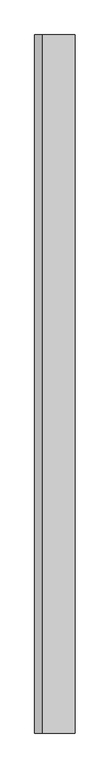
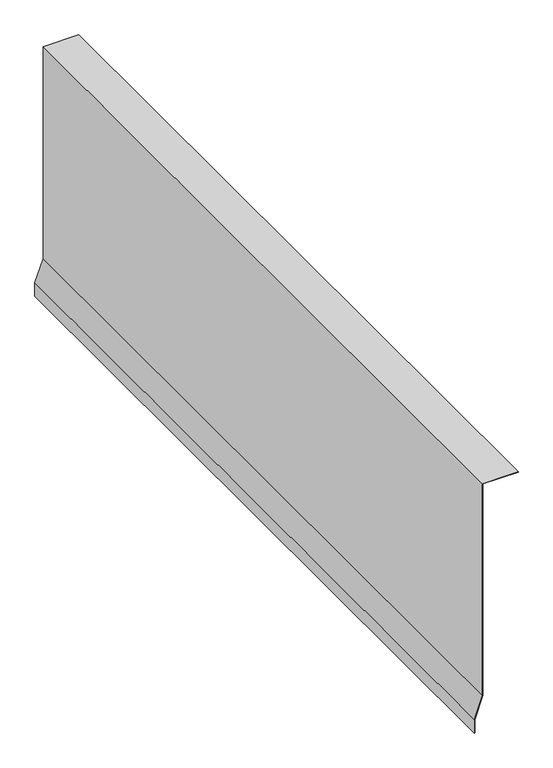
"""IFC4 building model written with IfcOpenShell, lengths in millimetres: proxy geometry, Membrane056 15639 : Membrane056 15639."""

from ifc_helpers import new_model, si_unit, frame, origin, place, context, project, spatial, polyline, outline, extrude, source, transform, mapped, element, save


def generic_models_2c707389(model_context):
    return source(origin(), model_context, "Body", "SweptSolid", [
        extrude(outline(polyline([(40237.828125, -4904.6197981), (40237.828125, -4998.1919031), (39649.4031064, -4998.1919031), (39589.4778975, -5020.0028954), (39552.6918208, -5020.0028954), (39552.6918208, -5019.0028954), (39589.3015705, -5019.0028954), (39649.2267794, -4997.1919031), (40236.828125, -4997.1919031), (40236.828125, -4904.6197981), (40237.828125, -4904.6197981)])), frame((0.0, -1052.8906574, 0.0), z_axis=(0.0, 1.0, 0.0), x_axis=(0.0, 0.0, 1.0)), (0.0, 0.0, 1.0), 2000.0),
    ])


if __name__ == "__main__":
    model = new_model("IFC4")
    model_context = context("Model", 3, world=origin())
    ifc_project = project(units=[si_unit("LENGTHUNIT", "METRE", prefix="MILLI")], contexts=[model_context])
    site = spatial("IfcSite", under=ifc_project)
    building = spatial("IfcBuilding", under=site)
    placement = place(None, origin())
    generic_models_shape = generic_models_2c707389(model_context)
    element("IfcBuildingElementProxy", 1, Name="Membrane056 15639 : Membrane056 15639", ObjectType="Membrane056 15639 : Membrane056 15639", at=placement, inside=building, context=model_context, shape_type="MappedRepresentation", body=[
        mapped(generic_models_shape, transform((0.0, 0.0, 0.0), x_axis=(1.0, 0.0, 0.0), y_axis=(0.0, 1.0, 0.0), z_axis=(0.0, 0.0, 1.0))),
    ])
    save(model, "model.ifc")

# Revit data of these elements
# Type "Membrane056 15639 : Membrane056 15639"
#   NameOverride = "Membrane056"
# Element 1 (IfcBuildingElementProxy, "Membrane056 15639 : Membrane056 15639")
#   Materials on its faces: "(2) LAYERS OF ICE & WATER SHIELD (BITUTHANE) UNDER STUCCO"
# Materials
#   "(2) LAYERS OF ICE & WATER SHIELD (BITUTHANE) UNDER STUCCO": class "Unassigned", colour RGB 186 255 159, transparency 0, Cost = 0
